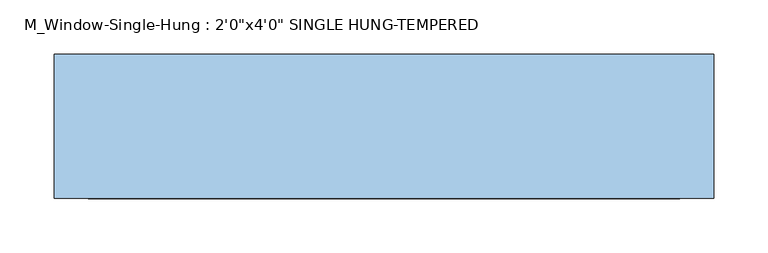
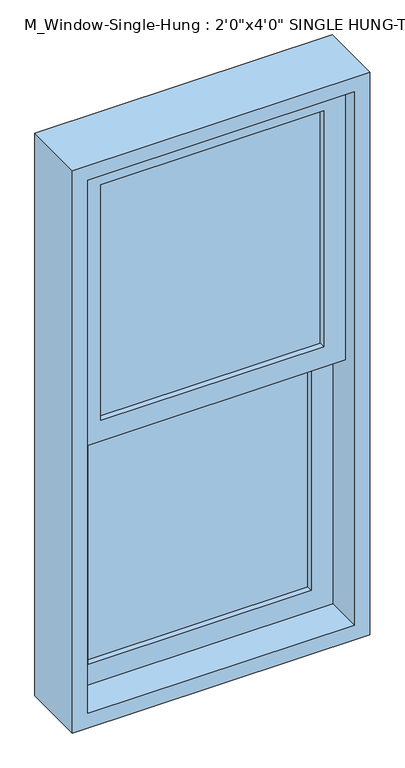
"""IFC4 building model written with IfcOpenShell, lengths in millimetres: window geometry."""

from ifc_helpers import new_model, si_unit, frame, origin, place, context, project, spatial, polyline, outline, extrude, source, transform, mapped, element, save


def window_73ce8039(model_context):
    return source(origin(), model_context, "Body", "SweptSolid", [
        extrude(outline(polyline([(228.6, 19.05), (-228.6, 19.05), (-228.6, 25.4), (228.6, 25.4), (228.6, 19.05)])), frame((0.0, 0.0, 990.6), z_axis=(0.0, 0.0, 1.0), x_axis=(1.0, 0.0, 0.0)), (0.0, 0.0, 1.0), 511.175),
        extrude(outline(polyline([(-228.6, 31.75), (-228.6, 38.1), (228.6, 38.1), (228.6, 31.75), (-228.6, 31.75)])), frame((0.0, 0.0, 990.6), z_axis=(0.0, 0.0, 1.0), x_axis=(1.0, 0.0, 0.0)), (0.0, 0.0, 1.0), 511.175),
        extrude(outline(polyline([(228.6, -25.4), (-228.6, -25.4), (-228.6, -19.05), (228.6, -19.05), (228.6, -25.4)])), frame((0.0, 0.0, 1546.225), z_axis=(0.0, 0.0, 1.0), x_axis=(1.0, 0.0, 0.0)), (0.0, 0.0, 1.0), 511.175),
        extrude(outline(polyline([(-228.6, -12.7), (-228.6, -6.35), (228.6, -6.35), (228.6, -12.7), (-228.6, -12.7)])), frame((0.0, 0.0, 1546.225), z_axis=(0.0, 0.0, 1.0), x_axis=(1.0, 0.0, 0.0)), (0.0, 0.0, 1.0), 511.175),
        extrude(outline(polyline([(1546.225, 273.05), (1546.225, -273.05), (946.15, -273.05), (946.15, 273.05), (1546.225, 273.05)]), holes=[polyline([(1501.775, -228.6), (1501.775, 228.6), (990.6, 228.6), (990.6, -228.6), (1501.775, -228.6)])]), frame((0.0, 6.35, 0.0), z_axis=(0.0, 1.0, 0.0), x_axis=(0.0, 0.0, 1.0)), (0.0, 0.0, 1.0), 44.45),
        extrude(outline(polyline([(2101.85, 273.05), (2101.85, -273.05), (1501.775, -273.05), (1501.775, 273.05), (2101.85, 273.05)]), holes=[polyline([(2057.4, -228.6), (2057.4, 228.6), (1546.225, 228.6), (1546.225, -228.6), (2057.4, -228.6)])]), frame((0.0, -38.1, 0.0), z_axis=(0.0, 1.0, 0.0), x_axis=(0.0, 0.0, 1.0)), (0.0, 0.0, 1.0), 44.45),
        extrude(outline(polyline([(2133.6, 304.8), (2133.6, -304.8), (914.4, -304.8), (914.4, 304.8), (2133.6, 304.8)]), holes=[polyline([(2101.85, -273.05), (2101.85, 273.05), (946.15, 273.05), (946.15, -273.05), (2101.85, -273.05)])]), frame((0.0, -69.85, 0.0), z_axis=(0.0, 1.0, 0.0), x_axis=(0.0, 0.0, 1.0)), (0.0, 0.0, 1.0), 133.35),
    ])


if __name__ == "__main__":
    model = new_model("IFC4")
    model_context = context("Model", 3, world=origin())
    ifc_project = project(units=[si_unit("LENGTHUNIT", "METRE", prefix="MILLI")], contexts=[model_context])
    site = spatial("IfcSite", under=ifc_project)
    building = spatial("IfcBuilding", under=site)
    placement = place(None, origin())
    window_shape = window_73ce8039(model_context)
    element("IfcWindow", 1, ObjectType="M_Window-Single-Hung : 2'0\"x4'0\" SINGLE HUNG-TEMPERED", at=placement, inside=building, context=model_context, shape_type="MappedRepresentation", body=[
        mapped(window_shape, transform((0.0, 0.0, 0.0), x_axis=(1.0, 0.0, 0.0), y_axis=(0.0, 1.0, 0.0), z_axis=(0.0, 0.0, 1.0))),
    ])
    save(model, "model.ifc")

# Revit data of these elements
# Type "M_Window-Single-Hung : 2'0\"x4'0\" SINGLE HUNG-TEMPERED"
#   Type Mark = "2"
#   Fire Rating = "0.5h"
#   Construction Type Id = "DG-DR"
#   Assembly Code = "B2020100"
#   Analytic Construction = "Double glazing - domestic"
#   Wall Thickness [instance default] = 0' - 5.90551"
#   Window Inset [instance default] = 0' - 0"
#   Visual Light Transmittance = 0.81
#   Thermal Resistance (R) = 1.8146 (h·ft²·°F)/BTU
#   Solar Heat Gain Coefficient = 0.76
#   Muntin Width = 1' - 6"
#   Muntin Height = 1' - 8 1/8"
#   Interior Wall Closure [instance default] = 0' - 1.40551"
#   Rough Width = 2' - 0.59055"
#   Rough Height = 4' - 0.59055"
#   Frame Extension [instance default] = 0' - 1 1/4"
#   Exterior Wall Closure [instance default] = 0' - 0 1/2"
#   Extension Jamb [instance default] = 0' - 1.40551"
#   Heat Transfer Coefficient (U) = 0.5511 BTU/(h·ft²·°F)
#   Height = 4' - 0"
#   Width = 2' - 0"
#   Top Muntin Visibility = yes
#   Indicator Visibility [instance default] = yes
#   Extension Jamb Visibility [instance default] = yes
#   Interior Trim Visibility [instance default] = yes
#   Exterior Trim Visibility [instance default] = yes
#   Define Thermal Properties by = 1
#   Bottom Muntin Visibility = yes
#   Muntin Pattern = M_Muntin Pattern_2x2 : M_Muntin Pattern_2x2
#   Interior Trim Material = Wood - Stained
#   Interior Trim = M_Trim-Window-Interior-Flat : Picture Frame
#   Exterior Trim Material = Clad - White
#   Exterior Trim = M_Trim-Window-Exterior-Flat : with Sill
#   Glass Panel Material = Glass
#   Exterior Frame Material = Clad - White
#   Interior Frame Material = Wood - Stained
#   Wall Closure = (empty or 0)
# Element 1 (IfcWindow, "M_Window-Single-Hung : 2'0\"x4'0\" SINGLE HUNG-TEMPERED")
#   Wall Thickness = 0' - 4"
#   Extension Jamb = 0' - 1"
#   Extension Jamb Visibility = no
#   Materials on its faces: "Wood - Stained", "Glass", "Clad - White"
# Materials
#   "Wood - Stained": class "Wood", colour RGB 224 178 126, transparency 0, Cost = 0
#   "Clad - White": class "Wood", colour RGB 242 242 238, transparency 0, Cost = 0
#   "Glass": class "Glass", colour RGB 0 128 192, transparency 0.75, Description = "Soda Lime Glass", Cost = 0
